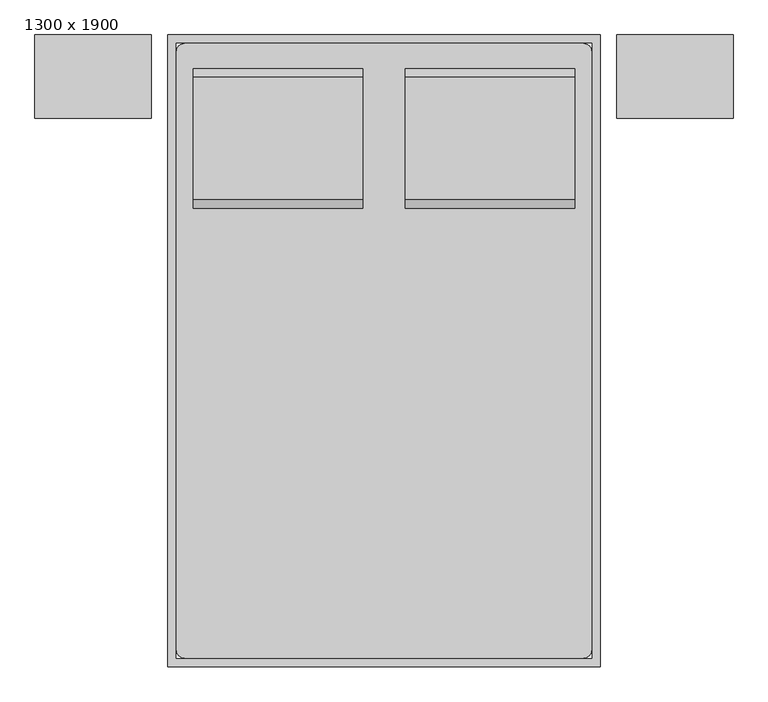
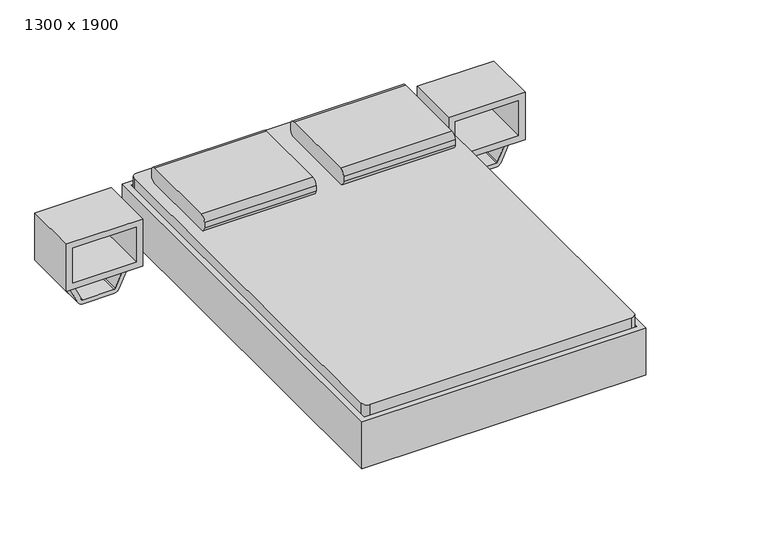
"""IFC4 building model written with IfcOpenShell, lengths in millimetres: furniture geometry, 双人床带床头柜 : 1300 x 1900."""

import ifcopenshell
import ifcopenshell.guid

model = None  # the IFC model being written
_history = None  # IfcOwnerHistory: only IFC2X3 demands one
_inside = {}  # id of a spatial element -> (the spatial element, [elements in it])
_under = {}  # id of a project, library or spatial element -> (it, [spatial elements below it])
_declared = {}  # id of a project -> (the project, [libraries it declares])
_typed = {}  # id of a type object -> (the type object, [elements of that type])
_made_of = {}  # id of a material, layer set ... -> (it, [elements and type objects made of it])


def new_model(schema):
    """Start an empty IFC model of exactly this schema.

    Asked for "IFC4X3", IfcOpenShell would pick the latest addendum, in which some entities
    have other attributes; the version numbers below select the first issue.
    IFC2X3 requires an IfcOwnerHistory on every rooted entity: one is made here for all.
    """
    global model, _history
    if schema == "IFC4X3":
        model = ifcopenshell.file(schema_version=(4, 3, 0, 0))
    else:
        model = ifcopenshell.file(schema=schema)
    _inside.clear()
    _under.clear()
    _declared.clear()
    _typed.clear()
    _made_of.clear()
    _history = None
    if model.schema == "IFC2X3":
        org = make("IfcOrganization", Name="unknown")
        user = make(
            "IfcPersonAndOrganization",
            ThePerson=make("IfcPerson", FamilyName="unknown"),
            TheOrganization=org,
        )
        app = make(
            "IfcApplication",
            ApplicationDeveloper=org,
            Version="unknown",
            ApplicationFullName="unknown",
            ApplicationIdentifier="unknown",
        )
        _history = make(
            "IfcOwnerHistory",
            OwningUser=user,
            OwningApplication=app,
            ChangeAction="ADDED",
            CreationDate=0,
        )
    return model


def make(cls, **values):
    """One entity of the class cls with the attributes given. An attribute that is None is left unset."""
    return model.create_entity(
        cls, **{name: value for name, value in values.items() if value is not None}
    )


def rooted(cls, **values):
    """An entity with a GlobalId (a new one), such as an element, a storey or a relation."""
    return make(cls, GlobalId=ifcopenshell.guid.new(), OwnerHistory=_history, **values)


def si_unit(unit_type, name, prefix=None):
    """IfcSIUnit, for example si_unit("LENGTHUNIT", "METRE", prefix="MILLI")."""
    return make("IfcSIUnit", UnitType=unit_type, Prefix=prefix, Name=name)


def assignment(units):
    """IfcUnitAssignment: the units of a project."""
    return None if units is None else make("IfcUnitAssignment", Units=units)


def point(xyz):
    """IfcCartesianPoint."""
    return None if xyz is None else make("IfcCartesianPoint", Coordinates=xyz)


def direction(xyz):
    """IfcDirection."""
    return None if xyz is None else make("IfcDirection", DirectionRatios=xyz)


def frame(location, z_axis=None, x_axis=None):
    """IfcAxis2Placement3D, a coordinate frame: its origin and axes. An axis left out is left unset."""
    return make(
        "IfcAxis2Placement3D",
        Location=point(location),
        Axis=direction(z_axis),
        RefDirection=direction(x_axis),
    )


def frame_2d(location, x_axis=None):
    """IfcAxis2Placement2D, a coordinate frame in the plane: its origin and x axis."""
    return make(
        "IfcAxis2Placement2D", Location=point(location), RefDirection=direction(x_axis)
    )


def origin():
    """The frame at (0, 0, 0) with its axes left unset."""
    return frame((0.0, 0.0, 0.0))


def place(relative_to, where):
    """IfcLocalPlacement: puts the frame where relative to a parent placement (None: the world)."""
    return make(
        "IfcLocalPlacement", PlacementRelTo=relative_to, RelativePlacement=where
    )


def context(
    kind, dimensions, precision=None, world=None, true_north=None, identifier=None
):
    """IfcGeometricRepresentationContext, for example the 3D "Model" context."""
    return make(
        "IfcGeometricRepresentationContext",
        ContextIdentifier=identifier,
        ContextType=kind,
        CoordinateSpaceDimension=dimensions,
        Precision=precision,
        WorldCoordinateSystem=world,
        TrueNorth=true_north,
    )


def project(units=None, contexts=None):
    """IfcProject with its units and contexts."""
    return rooted(
        "IfcProject",
        Name="project",
        RepresentationContexts=contexts,
        UnitsInContext=assignment(units),
    )


def spatial(cls, under=None, at=None, **own):
    """A site, building, storey or space (cls), placed at a placement, below another one or the project."""
    s = rooted(cls, ObjectPlacement=at, **own)
    if under is not None:
        _under.setdefault(under.id(), (under, []))[1].append(s)
    return s


def polyline(points):
    """IfcPolyline through the points."""
    return make("IfcPolyline", Points=[point(p) for p in points])


def circle_curve(where, radius):
    """IfcCircle in the frame where."""
    return make("IfcCircle", Position=where, Radius=radius)


def trimmed(basis, trim1, trim2, sense, master):
    """IfcTrimmedCurve: the piece of a basis curve between two trims."""
    return make(
        "IfcTrimmedCurve",
        BasisCurve=basis,
        Trim1=trim1,
        Trim2=trim2,
        SenseAgreement=sense,
        MasterRepresentation=master,
    )


def segment(curve, same_sense, transition):
    """IfcCompositeCurveSegment."""
    return make(
        "IfcCompositeCurveSegment",
        Transition=transition,
        SameSense=same_sense,
        ParentCurve=curve,
    )


def composite_curve(segments, self_intersect=None):
    """IfcCompositeCurve: segments joined end to end."""
    return make("IfcCompositeCurve", Segments=segments, SelfIntersect=self_intersect)


def outline(outer, holes=None, kind="AREA"):
    """IfcArbitraryClosedProfileDef: a profile drawn as a closed curve; with holes, ...WithVoids."""
    if holes is None:
        return make("IfcArbitraryClosedProfileDef", ProfileType=kind, OuterCurve=outer)
    return make(
        "IfcArbitraryProfileDefWithVoids",
        ProfileType=kind,
        OuterCurve=outer,
        InnerCurves=holes,
    )


def extrude(swept, where, along, depth):
    """IfcExtrudedAreaSolid: the profile swept, set in the frame where, extruded along a direction by depth."""
    return make(
        "IfcExtrudedAreaSolid",
        SweptArea=swept,
        Position=where,
        ExtrudedDirection=direction(along),
        Depth=depth,
    )


def shape(context_of_items, identifier, shape_type, items):
    """IfcShapeRepresentation: the items that make up one representation, for example the "Body"."""
    return make(
        "IfcShapeRepresentation",
        ContextOfItems=context_of_items,
        RepresentationIdentifier=identifier,
        RepresentationType=shape_type,
        Items=items,
    )


def source(mapping_origin, context_of_items, identifier, shape_type, items):
    """IfcRepresentationMap: a shape defined once, which mapped items show again and again."""
    return make(
        "IfcRepresentationMap",
        MappingOrigin=mapping_origin,
        MappedRepresentation=shape(context_of_items, identifier, shape_type, items),
    )


def transform(
    local_origin,
    x_axis=None,
    y_axis=None,
    z_axis=None,
    scale=None,
    scale2=None,
    scale3=None,
    uniform=True,
):
    """IfcCartesianTransformationOperator3D, or its non-uniform kind. x_axis, y_axis, z_axis: its Axis1, 2, 3."""
    if uniform:
        return make(
            "IfcCartesianTransformationOperator3D",
            Axis1=direction(x_axis),
            Axis2=direction(y_axis),
            LocalOrigin=point(local_origin),
            Scale=scale,
            Axis3=direction(z_axis),
        )
    return make(
        "IfcCartesianTransformationOperator3DnonUniform",
        Axis1=direction(x_axis),
        Axis2=direction(y_axis),
        LocalOrigin=point(local_origin),
        Scale=scale,
        Axis3=direction(z_axis),
        Scale2=scale2,
        Scale3=scale3,
    )


def mapped(mapping_source, mapping_target):
    """IfcMappedItem: shows the shape of a source again, moved by a transform."""
    return make(
        "IfcMappedItem", MappingSource=mapping_source, MappingTarget=mapping_target
    )


def made_of(thing, what):
    """Note that an element or type object is made of a material, layer set ...; save() writes the relation."""
    if what is not None:
        _made_of.setdefault(what.id(), (what, []))[1].append(thing)
    return thing


def element(
    cls,
    number,
    at=None,
    inside=None,
    cuts=None,
    type_object=None,
    material=None,
    context=None,
    identifier="Body",
    shape_type=None,
    held_by="IfcProductDefinitionShape",
    body=None,
    shapes=None,
    **own,
):
    """One element of the class cls, such as IfcWall. Its Tag is "e" and its number.

    at: its placement. inside: the storey or other place that contains it. cuts: it is an
    opening in that element (IfcRelVoidsElement). A single representation is given by context,
    identifier, shape_type and body (its items); several are given by shapes. held_by: the class
    of the entity that holds the representations. save() writes the other relations.
    """
    e = rooted(cls, Tag="e%d" % number, ObjectPlacement=at, **own)
    if body is not None:
        shapes = [shape(context, identifier, shape_type, body)]
    if shapes is not None:
        e.Representation = make(held_by, Representations=shapes)
    if inside is not None:
        _inside.setdefault(inside.id(), (inside, []))[1].append(e)
    if cuts is not None:
        rooted(
            "IfcRelVoidsElement", RelatingBuildingElement=cuts, RelatedOpeningElement=e
        )
    if type_object is not None:
        _typed.setdefault(type_object.id(), (type_object, []))[1].append(e)
    return made_of(e, material)


def aggregate(whole, parts):
    """IfcRelAggregates: a whole, such as a stair, and the parts it consists of."""
    return rooted("IfcRelAggregates", RelatingObject=whole, RelatedObjects=parts)


def save(model, path):
    """Write the relations noted so far, then the file.

    IfcRelAggregates (storeys below a building ...), IfcRelContainedInSpatialStructure (elements
    in a storey), IfcRelDefinesByType, IfcRelAssociatesMaterial and IfcRelDeclares: one each for
    every whole, place, type object, material and project.
    """
    for whole, parts in _under.values():
        aggregate(whole, parts)
    for where, things in _inside.values():
        rooted(
            "IfcRelContainedInSpatialStructure",
            RelatedElements=things,
            RelatingStructure=where,
        )
    for kind, things in _typed.values():
        rooted("IfcRelDefinesByType", RelatedObjects=things, RelatingType=kind)
    for what, things in _made_of.values():
        rooted("IfcRelAssociatesMaterial", RelatedObjects=things, RelatingMaterial=what)
    for by, libraries in _declared.values():
        rooted("IfcRelDeclares", RelatingContext=by, RelatedDefinitions=libraries)
    model.write(path)


def plane_surface(at):
    """IfcPlane: the flat surface through the origin of the frame at, square to its z axis."""
    return make("IfcPlane", Position=at)


def cylinder_surface(at, radius):
    """IfcCylindricalSurface: all points at the distance radius from the z axis of the frame at."""
    return make("IfcCylindricalSurface", Position=at, Radius=radius)


def revolved_surface(curve, axis_point, axis_direction):
    """IfcSurfaceOfRevolution: the curve turned about the line through axis_point along axis_direction."""
    return make(
        "IfcSurfaceOfRevolution",
        SweptCurve=make("IfcArbitraryOpenProfileDef", ProfileType="CURVE", Curve=curve),
        AxisPosition=make("IfcAxis1Placement", Location=point(axis_point), Axis=direction(axis_direction)),
    )


def advanced_brep(points, edges, surfaces, faces):
    """IfcAdvancedBrep: a solid bounded by faces that lie on surfaces and meet in shared edges.

    An edge is (start, end): straight between two places in points (the first is 0);
    or (start, end, curve); or (start, end, curve, False) where it runs against its curve.
    A face is (place in surfaces, loops), or (place, loops, False) where it looks against
    its surface's normal. A loop lists edges by number (the first is 1), with a minus sign
    where the edge is run from its end to its start. The first loop is the outer one.
    """
    corners = [point(p) for p in points]
    vertices = [make("IfcVertexPoint", VertexGeometry=c) for c in corners]
    made = []
    for start, end, *more in edges:
        made.append(
            make(
                "IfcEdgeCurve",
                EdgeStart=vertices[start],
                EdgeEnd=vertices[end],
                EdgeGeometry=more[0] if more else make("IfcPolyline", Points=[corners[start], corners[end]]),
                SameSense=more[1] if len(more) > 1 else True,
            )
        )
    hull = []
    for where, loops, *sense in faces:
        bounds = []
        for j, loop in enumerate(loops):
            ring = [make("IfcOrientedEdge", EdgeElement=made[abs(k) - 1], Orientation=k > 0) for k in loop]
            bounds.append(
                make(
                    "IfcFaceOuterBound" if j == 0 else "IfcFaceBound",
                    Bound=make("IfcEdgeLoop", EdgeList=ring),
                    Orientation=True,
                )
            )
        hull.append(make("IfcAdvancedFace", Bounds=bounds, FaceSurface=surfaces[where], SameSense=sense[0] if sense else True))
    return make("IfcAdvancedBrep", Outer=make("IfcClosedShell", CfsFaces=hull))


def furniture_1300_x_1900_48583a1e(model_context):
    return source(origin(), model_context, "Body", "SolidModel", [
        advanced_brep(
        [(-285.1231784, 461.5704918, 177.8), (-285.1231784, 385.3704918, 177.8), (-285.1231784, 385.3704918, 196.85), (-285.1231784, 461.5704918, 196.85), (-234.3231784, 461.5704918, 177.8), (-234.3231784, 385.3704918, 177.8), (-222.1869899, 385.3704918, 196.85), (-222.1869899, 461.5704918, 196.85), (-158.2523099, 461.5704918, 14.6654962), (-158.2523099, 385.3704918, 14.6654962), (-140.9871466, 385.3704918, 22.716374), (-140.9871466, 461.5704918, 22.716374), (-135.2320921, 385.3704918, 0.0), (-135.2320921, 461.5704918, 0.0), (-135.2320921, 385.3704918, 19.05), (-135.2320921, 461.5704918, 19.05), (-56.6195862, 461.5704918, 0.0), (-56.6195862, 385.3704918, 0.0), (-56.6195862, 385.3704918, 19.05), (-56.6195862, 461.5704918, 19.05), (-43.9195862, 385.3704918, 3.4029547), (-43.9195862, 461.5704918, 3.4029547), (-53.4445862, 385.3704918, 19.9007387), (-53.4445862, 461.5704918, 19.9007387), (16.177459, 461.5704918, 38.1), (16.177459, 385.3704918, 38.1), (11.0730269, 385.3704918, 57.15), (11.0730269, 461.5704918, 57.15), (662.4518216, 461.5704918, 38.1), (662.4518216, 385.3704918, 38.1), (667.5562537, 385.3704918, 57.15), (667.5562537, 461.5704918, 57.15), (722.5488669, 461.5704918, 3.4029547), (722.5488669, 385.3704918, 3.4029547), (732.0738669, 385.3704918, 19.9007387), (732.0738669, 461.5704918, 19.9007387), (735.2488669, 385.3704918, 0.0), (735.2488669, 461.5704918, 0.0), (735.2488669, 385.3704918, 19.05), (735.2488669, 461.5704918, 19.05), (813.8613728, 461.5704918, 0.0), (813.8613728, 385.3704918, 0.0), (813.8613728, 385.3704918, 19.05), (813.8613728, 461.5704918, 19.05), (836.8815906, 385.3704918, 14.6654962), (836.8815906, 461.5704918, 14.6654962), (819.6164272, 385.3704918, 22.716374), (819.6164272, 461.5704918, 22.716374), (912.952459, 461.5704918, 177.8), (912.952459, 385.3704918, 177.8), (900.8162705, 385.3704918, 196.85), (900.8162705, 461.5704918, 196.85), (963.752459, 461.5704918, 177.8), (963.752459, 461.5704918, 196.85), (963.752459, 385.3704918, 196.85), (963.752459, 385.3704918, 177.8)],
        [
            (0, 1),
            (1, 2),
            (2, 3),
            (3, 0),
            (0, 4),
            (4, 5),
            (5, 1),
            (5, 6),
            (6, 2),
            (6, 7),
            (7, 3),
            (7, 4),
            (4, 8),
            (8, 9),
            (9, 5),
            (9, 10),
            (10, 6),
            (10, 11),
            (11, 7),
            (11, 8),
            (12, 9, circle_curve(frame((-135.2320921, 385.3704918, 25.4), z_axis=(0.0, 1.0, 0.0), x_axis=(-0.9063077870366494, 0.0, -0.4226182617407007)), 25.4)),
            (8, 13, circle_curve(frame((-135.2320921, 461.5704918, 25.4), z_axis=(0.0, -1.0, 0.0), x_axis=(-0.9063077870366494, 0.0, -0.4226182617407007)), 25.4)),
            (13, 12),
            (14, 10, circle_curve(frame((-135.2320921, 385.3704918, 25.4), z_axis=(0.0, 1.0, 0.0), x_axis=(-0.9063077870366494, 0.0, -0.4226182617407007)), 6.35)),
            (12, 14),
            (15, 11, circle_curve(frame((-135.2320921, 461.5704918, 25.4), z_axis=(0.0, 1.0, 0.0), x_axis=(-0.9063077870366494, 0.0, -0.4226182617407007)), 6.35)),
            (14, 15),
            (15, 13),
            (13, 16),
            (16, 17),
            (17, 12),
            (17, 18),
            (18, 14),
            (18, 19),
            (19, 15),
            (19, 16),
            (20, 17, circle_curve(frame((-56.6195862, 385.3704918, 25.4), z_axis=(0.0, 1.0, 0.0), x_axis=(0.0, 0.0, -1.0)), 25.4)),
            (16, 21, circle_curve(frame((-56.6195862, 461.5704918, 25.4), z_axis=(0.0, -1.0, 0.0), x_axis=(0.0, 0.0, -1.0)), 25.4)),
            (21, 20),
            (22, 18, circle_curve(frame((-56.6195862, 385.3704918, 25.4), z_axis=(0.0, 1.0, 0.0), x_axis=(0.0, 0.0, -1.0)), 6.35)),
            (20, 22),
            (23, 19, circle_curve(frame((-56.6195862, 461.5704918, 25.4), z_axis=(0.0, 1.0, 0.0), x_axis=(0.0, 0.0, -1.0)), 6.35)),
            (22, 23),
            (23, 21),
            (21, 24),
            (24, 25),
            (25, 20),
            (25, 26),
            (26, 22),
            (26, 27),
            (27, 23),
            (27, 24),
            (24, 28),
            (28, 29),
            (29, 25),
            (29, 30),
            (30, 26),
            (30, 31),
            (31, 27),
            (31, 28),
            (28, 32),
            (32, 33),
            (33, 29),
            (33, 34),
            (34, 30),
            (34, 35),
            (35, 31),
            (35, 32),
            (36, 33, circle_curve(frame((735.2488669, 385.3704918, 25.4), z_axis=(0.0, 1.0, 0.0), x_axis=(-0.5000000000000505, 0.0, -0.8660254037844094)), 25.4)),
            (32, 37, circle_curve(frame((735.2488669, 461.5704918, 25.4), z_axis=(0.0, -1.0, 0.0), x_axis=(-0.5000000000000505, 0.0, -0.8660254037844094)), 25.4)),
            (37, 36),
            (38, 34, circle_curve(frame((735.2488669, 385.3704918, 25.4), z_axis=(0.0, 1.0, 0.0), x_axis=(-0.5000000000000505, 0.0, -0.8660254037844094)), 6.35)),
            (36, 38),
            (39, 35, circle_curve(frame((735.2488669, 461.5704918, 25.4), z_axis=(0.0, 1.0, 0.0), x_axis=(-0.5000000000000505, 0.0, -0.8660254037844094)), 6.35)),
            (38, 39),
            (39, 37),
            (37, 40),
            (40, 41),
            (41, 36),
            (41, 42),
            (42, 38),
            (42, 43),
            (43, 39),
            (43, 40),
            (44, 41, circle_curve(frame((813.8613728, 385.3704918, 25.4), z_axis=(0.0, 1.0, 0.0), x_axis=(0.0, 0.0, -1.0)), 25.4)),
            (40, 45, circle_curve(frame((813.8613728, 461.5704918, 25.4), z_axis=(0.0, -1.0, 0.0), x_axis=(0.0, 0.0, -1.0)), 25.4)),
            (45, 44),
            (46, 42, circle_curve(frame((813.8613728, 385.3704918, 25.4), z_axis=(0.0, 1.0, 0.0), x_axis=(0.0, 0.0, -1.0)), 6.35)),
            (44, 46),
            (47, 43, circle_curve(frame((813.8613728, 461.5704918, 25.4), z_axis=(0.0, 1.0, 0.0), x_axis=(0.0, 0.0, -1.0)), 6.35)),
            (46, 47),
            (47, 45),
            (45, 48),
            (48, 49),
            (49, 44),
            (49, 50),
            (50, 46),
            (50, 51),
            (51, 47),
            (51, 48),
            (52, 53),
            (53, 54),
            (54, 55),
            (55, 52),
            (48, 52),
            (55, 49),
            (54, 50),
            (53, 51),
        ],
        [
            plane_surface(frame((-285.1231784, 715.5704918, -152.9490627), z_axis=(-1.0, 0.0, 0.0), x_axis=(0.0, 1.0, 0.0))),
            plane_surface(frame((-285.1231784, 461.5704918, 177.8), z_axis=(0.0, 0.0, -1.0), x_axis=(1.0, 0.0, 0.0))),
            plane_surface(frame((-285.1231784, 385.3704918, 177.8), z_axis=(0.0, -1.0, 0.0), x_axis=(1.0, 0.0, 0.0))),
            plane_surface(frame((-285.1231784, 385.3704918, 196.85), z_axis=(0.0, 0.0, 1.0), x_axis=(1.0, 0.0, 0.0))),
            plane_surface(frame((-285.1231784, 461.5704918, 196.85), z_axis=(0.0, 1.0, 0.0), x_axis=(1.0, 0.0, 0.0))),
            plane_surface(frame((-234.3231784, 461.5704918, 177.8), z_axis=(-0.9063077870366483, 0.0, -0.42261826174070305), x_axis=(0.42261826174070305, 0.0, -0.9063077870366483))),
            plane_surface(frame((-234.3231784, 385.3704918, 177.8), z_axis=(0.0, -1.0, 0.0), x_axis=(0.4226182617407031, 0.0, -0.9063077870366483))),
            plane_surface(frame((-222.1869899, 385.3704918, 196.85), z_axis=(0.9063077870366483, 0.0, 0.42261826174070316), x_axis=(0.42261826174070316, 0.0, -0.9063077870366483))),
            plane_surface(frame((-222.1869899, 461.5704918, 196.85), z_axis=(0.0, 1.0, 0.0), x_axis=(0.42261826174070316, 0.0, -0.9063077870366483))),
            cylinder_surface(frame((-135.2320921, 715.5704918, 25.4), z_axis=(0.0, -1.0, 0.0), x_axis=(-0.9063077870366494, 0.0, -0.4226182617407007)), 25.4),
            plane_surface(frame((-135.2320921, 385.3704918, 25.4), z_axis=(0.0, -1.0, 0.0), x_axis=(-0.9063077870366494, 0.0, -0.4226182617407007))),
            revolved_surface(polyline([(-140.9871465476827, 385.3704918, 22.71637403794655), (-140.9871465476827, 461.5704918, 22.71637403794655)]), (-135.2320921, 715.5704918, 25.4), (0.0, -1.0, 0.0)),
            plane_surface(frame((-135.2320921, 461.5704918, 25.4), z_axis=(0.0, 1.0, 0.0), x_axis=(-0.9063077870366494, 0.0, -0.4226182617407007))),
            plane_surface(frame((-135.2320921, 461.5704918, 0.0), z_axis=(0.0, 0.0, -1.0), x_axis=(1.0, 0.0, 0.0))),
            plane_surface(frame((-135.2320921, 385.3704918, 0.0), z_axis=(0.0, -1.0, 0.0), x_axis=(1.0, 0.0, 0.0))),
            plane_surface(frame((-135.2320921, 385.3704918, 19.05), z_axis=(0.0, 0.0, 1.0), x_axis=(1.0, 0.0, 0.0))),
            plane_surface(frame((-135.2320921, 461.5704918, 19.05), z_axis=(0.0, 1.0, 0.0), x_axis=(1.0, 0.0, 0.0))),
            cylinder_surface(frame((-56.6195862, 715.5704918, 25.4), z_axis=(0.0, -1.0, 0.0), x_axis=(0.0, 0.0, -1.0)), 25.4),
            plane_surface(frame((-56.6195862, 385.3704918, 25.4), z_axis=(0.0, -1.0, 0.0), x_axis=(0.0, 0.0, -1.0))),
            revolved_surface(polyline([(-56.6195862, 385.3704918, 19.049999999999997), (-56.6195862, 461.5704918, 19.049999999999997)]), (-56.6195862, 715.5704918, 25.4), (0.0, -1.0, 0.0)),
            plane_surface(frame((-56.6195862, 461.5704918, 25.4), z_axis=(0.0, 1.0, 0.0), x_axis=(0.0, 0.0, -1.0))),
            plane_surface(frame((-43.9195862, 461.5704918, 3.4029547), z_axis=(0.49999999999987826, 0.0, -0.8660254037845089), x_axis=(0.8660254037845089, 0.0, 0.49999999999987826))),
            plane_surface(frame((-43.9195862, 385.3704918, 3.4029547), z_axis=(0.0, -1.0, 0.0), x_axis=(0.866025403784509, 0.0, 0.49999999999987815))),
            plane_surface(frame((-53.4445862, 385.3704918, 19.9007387), z_axis=(-0.49999999999987926, 0.0, 0.8660254037845083), x_axis=(0.8660254037845083, 0.0, 0.49999999999987926))),
            plane_surface(frame((-53.4445862, 461.5704918, 19.9007387), z_axis=(0.0, 1.0, 0.0), x_axis=(0.8660254037845087, 0.0, 0.4999999999998789))),
            plane_surface(frame((16.177459, 461.5704918, 38.1), z_axis=(0.0, 0.0, -1.0), x_axis=(1.0, 0.0, 0.0))),
            plane_surface(frame((16.177459, 385.3704918, 38.1), z_axis=(0.0, -1.0, 0.0), x_axis=(1.0, 0.0, 0.0))),
            plane_surface(frame((11.0730269, 385.3704918, 57.15), z_axis=(0.0, 0.0, 1.0), x_axis=(1.0, 0.0, 0.0))),
            plane_surface(frame((11.0730269, 461.5704918, 57.15), z_axis=(0.0, 1.0, 0.0), x_axis=(1.0, 0.0, 0.0))),
            plane_surface(frame((662.4518216, 461.5704918, 38.1), z_axis=(-0.5000000000000518, 0.0, -0.8660254037844087), x_axis=(0.8660254037844087, 0.0, -0.5000000000000518))),
            plane_surface(frame((662.4518216, 385.3704918, 38.1), z_axis=(0.0, -1.0, 0.0), x_axis=(0.8660254037844093, 0.0, -0.500000000000051))),
            plane_surface(frame((667.5562537, 385.3704918, 57.15), z_axis=(0.5000000000000507, 0.0, 0.8660254037844094), x_axis=(0.8660254037844094, 0.0, -0.5000000000000507))),
            plane_surface(frame((667.5562537, 461.5704918, 57.15), z_axis=(0.0, 1.0000000000000002, 0.0), x_axis=(0.8660254037844094, 0.0, -0.5000000000000508))),
            cylinder_surface(frame((735.2488669, 715.5704918, 25.4), z_axis=(0.0, -1.0, 0.0), x_axis=(-0.5000000000000505, 0.0, -0.8660254037844094)), 25.4),
            plane_surface(frame((735.2488669, 385.3704918, 25.4), z_axis=(0.0, -1.0, 0.0), x_axis=(-0.5000000000000506, 0.0, -0.8660254037844095))),
            revolved_surface(polyline([(732.0738668999998, 385.3704918, 19.900738685969), (732.0738668999998, 461.5704918, 19.900738685969)]), (735.2488669, 715.5704918, 25.4), (0.0, -1.0, 0.0)),
            plane_surface(frame((735.2488669, 461.5704918, 25.4), z_axis=(0.0, 1.0, 0.0), x_axis=(-0.5000000000000506, 0.0, -0.8660254037844095))),
            plane_surface(frame((735.2488669, 461.5704918, 0.0), z_axis=(0.0, 0.0, -1.0), x_axis=(1.0, 0.0, 0.0))),
            plane_surface(frame((735.2488669, 385.3704918, 0.0), z_axis=(0.0, -1.0, 0.0), x_axis=(1.0, 0.0, 0.0))),
            plane_surface(frame((735.2488669, 385.3704918, 19.05), z_axis=(0.0, 0.0, 1.0), x_axis=(1.0, 0.0, 0.0))),
            plane_surface(frame((735.2488669, 461.5704918, 19.05), z_axis=(0.0, 1.0, 0.0), x_axis=(1.0, 0.0, 0.0))),
            cylinder_surface(frame((813.8613728, 715.5704918, 25.4), z_axis=(0.0, -1.0, 0.0), x_axis=(0.0, 0.0, -1.0)), 25.4),
            plane_surface(frame((813.8613728, 385.3704918, 25.4), z_axis=(0.0, -1.0, 0.0), x_axis=(0.0, 0.0, -1.0))),
            revolved_surface(polyline([(813.8613728, 385.3704918, 19.049999999999997), (813.8613728, 461.5704918, 19.049999999999997)]), (813.8613728, 715.5704918, 25.4), (0.0, -1.0, 0.0)),
            plane_surface(frame((813.8613728, 461.5704918, 25.4), z_axis=(0.0, 1.0, 0.0), x_axis=(0.0, 0.0, -1.0))),
            plane_surface(frame((836.8815906, 461.5704918, 14.6654962), z_axis=(0.9063077870366775, 0.0, -0.42261826174064077), x_axis=(0.42261826174064077, 0.0, 0.9063077870366775))),
            plane_surface(frame((836.8815906, 385.3704918, 14.6654962), z_axis=(0.0, -1.0, 0.0), x_axis=(0.42261826174063993, 0.0, 0.9063077870366777))),
            plane_surface(frame((819.6164272, 385.3704918, 22.716374), z_axis=(-0.9063077870366776, 0.0, 0.4226182617406402), x_axis=(0.4226182617406402, 0.0, 0.9063077870366776))),
            plane_surface(frame((819.6164272, 461.5704918, 22.716374), z_axis=(0.0, 1.0, 0.0), x_axis=(0.4226182617406405, 0.0, 0.9063077870366775))),
            plane_surface(frame((963.752459, 715.5704918, -152.9490627), z_axis=(1.0, 0.0, 0.0), x_axis=(0.0, 1.0, 0.0))),
            plane_surface(frame((912.952459, 461.5704918, 177.8), z_axis=(0.0, 0.0, -1.0), x_axis=(1.0, 0.0, 0.0))),
            plane_surface(frame((912.952459, 385.3704918, 177.8), z_axis=(0.0, -1.0, 0.0), x_axis=(1.0, 0.0, 0.0))),
            plane_surface(frame((900.8162705, 385.3704918, 196.85), z_axis=(0.0, 0.0, 1.0), x_axis=(1.0, 0.0, 0.0))),
            plane_surface(frame((900.8162705, 461.5704918, 196.85), z_axis=(0.0, 1.0, 0.0), x_axis=(1.0, 0.0, 0.0))),
        ],
        [
            (0, [[1, 2, 3, 4]]),
            (1, [[-1, 5, 6, 7]]),
            (2, [[-2, -7, 8, 9]]),
            (3, [[-3, -9, 10, 11]]),
            (4, [[-4, -11, 12, -5]]),
            (5, [[-6, 13, 14, 15]]),
            (6, [[-8, -15, 16, 17]]),
            (7, [[-10, -17, 18, 19]]),
            (8, [[-12, -19, 20, -13]]),
            (9, [[21, -14, 22, 23]]),
            (10, [[24, -16, -21, 25]]),
            (11, [[26, -18, -24, 27]]),
            (12, [[-22, -20, -26, 28]]),
            (13, [[-23, 29, 30, 31]]),
            (14, [[-25, -31, 32, 33]]),
            (15, [[-27, -33, 34, 35]]),
            (16, [[-28, -35, 36, -29]]),
            (17, [[37, -30, 38, 39]]),
            (18, [[40, -32, -37, 41]]),
            (19, [[42, -34, -40, 43]]),
            (20, [[-38, -36, -42, 44]]),
            (21, [[-39, 45, 46, 47]]),
            (22, [[-41, -47, 48, 49]]),
            (23, [[-43, -49, 50, 51]]),
            (24, [[-44, -51, 52, -45]]),
            (25, [[-46, 53, 54, 55]]),
            (26, [[-48, -55, 56, 57]]),
            (27, [[-50, -57, 58, 59]]),
            (28, [[-52, -59, 60, -53]]),
            (29, [[-54, 61, 62, 63]]),
            (30, [[-56, -63, 64, 65]]),
            (31, [[-58, -65, 66, 67]]),
            (32, [[-60, -67, 68, -61]]),
            (33, [[69, -62, 70, 71]]),
            (34, [[72, -64, -69, 73]]),
            (35, [[74, -66, -72, 75]]),
            (36, [[-70, -68, -74, 76]]),
            (37, [[-71, 77, 78, 79]]),
            (38, [[-73, -79, 80, 81]]),
            (39, [[-75, -81, 82, 83]]),
            (40, [[-76, -83, 84, -77]]),
            (41, [[85, -78, 86, 87]]),
            (42, [[88, -80, -85, 89]]),
            (43, [[90, -82, -88, 91]]),
            (44, [[-86, -84, -90, 92]]),
            (45, [[-87, 93, 94, 95]]),
            (46, [[-89, -95, 96, 97]]),
            (47, [[-91, -97, 98, 99]]),
            (48, [[-92, -99, 100, -93]]),
            (49, [[101, 102, 103, 104]]),
            (50, [[-94, 105, -104, 106]]),
            (51, [[-96, -106, -103, 107]]),
            (52, [[-98, -107, -102, 108]]),
            (53, [[-100, -108, -101, -105]]),
        ],
    ),
        advanced_brep(
        [(-285.447541, -879.6295082, 196.85), (-285.447541, -879.6295082, 177.8), (-285.447541, -955.8295082, 177.8), (-285.447541, -955.8295082, 196.85), (-222.5113525, -879.6295082, 196.85), (-234.647541, -879.6295082, 177.8), (-234.647541, -955.8295082, 177.8), (-222.5113525, -955.8295082, 196.85), (-141.3115092, -879.6295082, 22.716374), (-158.5766725, -879.6295082, 14.6654962), (-158.5766725, -955.8295082, 14.6654962), (-141.3115092, -955.8295082, 22.716374), (-135.5564547, -879.6295082, 0.0), (-135.5564547, -879.6295082, 19.05), (-135.5564547, -955.8295082, 0.0), (-135.5564547, -955.8295082, 19.05), (-56.9439489, -879.6295082, 19.05), (-56.9439489, -879.6295082, 0.0), (-56.9439489, -955.8295082, 0.0), (-56.9439489, -955.8295082, 19.05), (-44.2439489, -879.6295082, 3.4029547), (-53.7689489, -879.6295082, 19.9007387), (-44.2439489, -955.8295082, 3.4029547), (-53.7689489, -955.8295082, 19.9007387), (10.7486643, -879.6295082, 57.15), (15.8530964, -879.6295082, 38.1), (15.8530964, -955.8295082, 38.1), (10.7486643, -955.8295082, 57.15), (667.5562537, -879.6295082, 57.15), (662.4518216, -879.6295082, 38.1), (662.4518216, -955.8295082, 38.1), (667.5562537, -955.8295082, 57.15), (732.0738669, -879.6295082, 19.9007387), (722.5488669, -879.6295082, 3.4029547), (722.5488669, -955.8295082, 3.4029547), (732.0738669, -955.8295082, 19.9007387), (735.2488669, -879.6295082, 0.0), (735.2488669, -879.6295082, 19.05), (735.2488669, -955.8295082, 0.0), (735.2488669, -955.8295082, 19.05), (813.8613728, -879.6295082, 19.05), (813.8613728, -879.6295082, 0.0), (813.8613728, -955.8295082, 0.0), (813.8613728, -955.8295082, 19.05), (836.8815906, -879.6295082, 14.6654962), (819.6164272, -879.6295082, 22.716374), (836.8815906, -955.8295082, 14.6654962), (819.6164272, -955.8295082, 22.716374), (900.8162705, -879.6295082, 196.85), (912.952459, -879.6295082, 177.8), (912.952459, -955.8295082, 177.8), (900.8162705, -955.8295082, 196.85), (963.752459, -879.6295082, 196.85), (963.752459, -955.8295082, 196.85), (963.752459, -955.8295082, 177.8), (963.752459, -879.6295082, 177.8)],
        [
            (0, 1),
            (1, 2),
            (2, 3),
            (3, 0),
            (0, 4),
            (4, 5),
            (5, 1),
            (5, 6),
            (6, 2),
            (6, 7),
            (7, 3),
            (7, 4),
            (4, 8),
            (8, 9),
            (9, 5),
            (9, 10),
            (10, 6),
            (10, 11),
            (11, 7),
            (11, 8),
            (12, 9, circle_curve(frame((-135.5564547, -879.6295082, 25.4), z_axis=(0.0, 1.0, 0.0), x_axis=(-0.9063077870366627, 0.0, -0.42261826174067213)), 25.4)),
            (8, 13, circle_curve(frame((-135.5564547, -879.6295082, 25.4), z_axis=(0.0, -1.0, 0.0), x_axis=(-0.9063077870366627, 0.0, -0.42261826174067213)), 6.35)),
            (13, 12),
            (14, 10, circle_curve(frame((-135.5564547, -955.8295082, 25.4), z_axis=(0.0, 1.0, 0.0), x_axis=(-0.9063077870366627, 0.0, -0.42261826174067213)), 25.4)),
            (12, 14),
            (15, 11, circle_curve(frame((-135.5564547, -955.8295082, 25.4), z_axis=(0.0, 1.0, 0.0), x_axis=(-0.9063077870366627, 0.0, -0.42261826174067213)), 6.35)),
            (14, 15),
            (15, 13),
            (13, 16),
            (16, 17),
            (17, 12),
            (17, 18),
            (18, 14),
            (18, 19),
            (19, 15),
            (19, 16),
            (20, 17, circle_curve(frame((-56.9439489, -879.6295082, 25.4), z_axis=(0.0, 1.0, 0.0), x_axis=(0.0, 0.0, -1.0)), 25.4)),
            (16, 21, circle_curve(frame((-56.9439489, -879.6295082, 25.4), z_axis=(0.0, -1.0, 0.0), x_axis=(0.0, 0.0, -1.0)), 6.35)),
            (21, 20),
            (22, 18, circle_curve(frame((-56.9439489, -955.8295082, 25.4), z_axis=(0.0, 1.0, 0.0), x_axis=(0.0, 0.0, -1.0)), 25.4)),
            (20, 22),
            (23, 19, circle_curve(frame((-56.9439489, -955.8295082, 25.4), z_axis=(0.0, 1.0, 0.0), x_axis=(0.0, 0.0, -1.0)), 6.35)),
            (22, 23),
            (23, 21),
            (21, 24),
            (24, 25),
            (25, 20),
            (25, 26),
            (26, 22),
            (26, 27),
            (27, 23),
            (27, 24),
            (24, 28),
            (28, 29),
            (29, 25),
            (29, 30),
            (30, 26),
            (30, 31),
            (31, 27),
            (31, 28),
            (28, 32),
            (32, 33),
            (33, 29),
            (33, 34),
            (34, 30),
            (34, 35),
            (35, 31),
            (35, 32),
            (36, 33, circle_curve(frame((735.2488669, -879.6295082, 25.4), z_axis=(0.0, 1.0, 0.0), x_axis=(-0.5000000000000517, 0.0, -0.8660254037844087)), 25.4)),
            (32, 37, circle_curve(frame((735.2488669, -879.6295082, 25.4), z_axis=(0.0, -1.0, 0.0), x_axis=(-0.5000000000000517, 0.0, -0.8660254037844087)), 6.35)),
            (37, 36),
            (38, 34, circle_curve(frame((735.2488669, -955.8295082, 25.4), z_axis=(0.0, 1.0, 0.0), x_axis=(-0.5000000000000517, 0.0, -0.8660254037844087)), 25.4)),
            (36, 38),
            (39, 35, circle_curve(frame((735.2488669, -955.8295082, 25.4), z_axis=(0.0, 1.0, 0.0), x_axis=(-0.5000000000000517, 0.0, -0.8660254037844087)), 6.35)),
            (38, 39),
            (39, 37),
            (37, 40),
            (40, 41),
            (41, 36),
            (41, 42),
            (42, 38),
            (42, 43),
            (43, 39),
            (43, 40),
            (44, 41, circle_curve(frame((813.8613728, -879.6295082, 25.4), z_axis=(0.0, 1.0, 0.0), x_axis=(0.0, 0.0, -1.0)), 25.4)),
            (40, 45, circle_curve(frame((813.8613728, -879.6295082, 25.4), z_axis=(0.0, -1.0, 0.0), x_axis=(0.0, 0.0, -1.0)), 6.35)),
            (45, 44),
            (46, 42, circle_curve(frame((813.8613728, -955.8295082, 25.4), z_axis=(0.0, 1.0, 0.0), x_axis=(0.0, 0.0, -1.0)), 25.4)),
            (44, 46),
            (47, 43, circle_curve(frame((813.8613728, -955.8295082, 25.4), z_axis=(0.0, 1.0, 0.0), x_axis=(0.0, 0.0, -1.0)), 6.35)),
            (46, 47),
            (47, 45),
            (45, 48),
            (48, 49),
            (49, 44),
            (49, 50),
            (50, 46),
            (50, 51),
            (51, 47),
            (51, 48),
            (52, 53),
            (53, 54),
            (54, 55),
            (55, 52),
            (48, 52),
            (55, 49),
            (54, 50),
            (53, 51),
        ],
        [
            plane_surface(frame((-285.447541, -1184.4295082, -127.5947323), z_axis=(-1.0, 0.0, 0.0), x_axis=(0.0, 1.0, 0.0))),
            plane_surface(frame((-285.447541, -879.6295082, 196.85), z_axis=(0.0, 1.0, 0.0), x_axis=(1.0, 0.0, 0.0))),
            plane_surface(frame((-285.447541, -879.6295082, 177.8), z_axis=(0.0, 0.0, -1.0), x_axis=(1.0, 0.0, 0.0))),
            plane_surface(frame((-285.447541, -955.8295082, 177.8), z_axis=(0.0, -1.0, 0.0), x_axis=(1.0, 0.0, 0.0))),
            plane_surface(frame((-285.447541, -955.8295082, 196.85), z_axis=(0.0, 0.0, 1.0), x_axis=(1.0, 0.0, 0.0))),
            plane_surface(frame((-222.5113525, -879.6295082, 196.85), z_axis=(0.0, 1.0, 0.0), x_axis=(0.42261826174067113, 0.0, -0.9063077870366631))),
            plane_surface(frame((-234.647541, -879.6295082, 177.8), z_axis=(-0.9063077870366633, 0.0, -0.422618261740671), x_axis=(0.422618261740671, 0.0, -0.9063077870366633))),
            plane_surface(frame((-234.647541, -955.8295082, 177.8), z_axis=(0.0, -1.0, 0.0), x_axis=(0.422618261740671, 0.0, -0.9063077870366633))),
            plane_surface(frame((-222.5113525, -955.8295082, 196.85), z_axis=(0.9063077870366631, 0.0, 0.42261826174067113), x_axis=(0.42261826174067113, 0.0, -0.9063077870366631))),
            plane_surface(frame((-135.5564547, -879.6295082, 25.4), z_axis=(0.0, 1.0, 0.0), x_axis=(-0.9063077870366627, 0.0, -0.42261826174067213))),
            cylinder_surface(frame((-135.5564547, -1184.4295082, 25.4), z_axis=(0.0, -1.0, 0.0), x_axis=(-0.9063077870366627, 0.0, -0.42261826174067213)), 25.4),
            plane_surface(frame((-135.5564547, -955.8295082, 25.4), z_axis=(0.0, -1.0, 0.0), x_axis=(-0.9063077870366627, 0.0, -0.42261826174067213))),
            revolved_surface(polyline([(-141.31150914768278, -955.8295082, 22.716374037946732), (-141.31150914768278, -879.6295082, 22.716374037946732)]), (-135.5564547, -1184.4295082, 25.4), (0.0, -1.0, 0.0)),
            plane_surface(frame((-135.5564547, -879.6295082, 19.05), z_axis=(0.0, 1.0, 0.0), x_axis=(1.0, 0.0, 0.0))),
            plane_surface(frame((-135.5564547, -879.6295082, 0.0), z_axis=(0.0, 0.0, -1.0), x_axis=(1.0, 0.0, 0.0))),
            plane_surface(frame((-135.5564547, -955.8295082, 0.0), z_axis=(0.0, -1.0, 0.0), x_axis=(1.0, 0.0, 0.0))),
            plane_surface(frame((-135.5564547, -955.8295082, 19.05), z_axis=(0.0, 0.0, 1.0), x_axis=(1.0, 0.0, 0.0))),
            plane_surface(frame((-56.9439489, -879.6295082, 25.4), z_axis=(0.0, 1.0, 0.0), x_axis=(0.0, 0.0, -1.0))),
            cylinder_surface(frame((-56.9439489, -1184.4295082, 25.4), z_axis=(0.0, -1.0, 0.0), x_axis=(0.0, 0.0, -1.0)), 25.4),
            plane_surface(frame((-56.9439489, -955.8295082, 25.4), z_axis=(0.0, -1.0, 0.0), x_axis=(0.0, 0.0, -1.0))),
            revolved_surface(polyline([(-56.9439489, -955.8295082, 19.049999999999997), (-56.9439489, -879.6295082, 19.049999999999997)]), (-56.9439489, -1184.4295082, 25.4), (0.0, -1.0, 0.0)),
            plane_surface(frame((-53.7689489, -879.6295082, 19.9007387), z_axis=(0.0, 1.0, 0.0), x_axis=(0.8660254037844793, 0.0, 0.4999999999999296))),
            plane_surface(frame((-44.2439489, -879.6295082, 3.4029547), z_axis=(0.4999999999999292, 0.0, -0.8660254037844796), x_axis=(0.8660254037844796, 0.0, 0.4999999999999292))),
            plane_surface(frame((-44.2439489, -955.8295082, 3.4029547), z_axis=(0.0, -1.0000000000000002, 0.0), x_axis=(0.8660254037844802, 0.0, 0.4999999999999281))),
            plane_surface(frame((-53.7689489, -955.8295082, 19.9007387), z_axis=(-0.49999999999992867, 0.0, 0.8660254037844798), x_axis=(0.8660254037844798, 0.0, 0.49999999999992867))),
            plane_surface(frame((10.7486643, -879.6295082, 57.15), z_axis=(0.0, 1.0, 0.0), x_axis=(1.0, 0.0, 0.0))),
            plane_surface(frame((15.8530964, -879.6295082, 38.1), z_axis=(0.0, 0.0, -1.0), x_axis=(1.0, 0.0, 0.0))),
            plane_surface(frame((15.8530964, -955.8295082, 38.1), z_axis=(0.0, -1.0, 0.0), x_axis=(1.0, 0.0, 0.0))),
            plane_surface(frame((10.7486643, -955.8295082, 57.15), z_axis=(0.0, 0.0, 1.0), x_axis=(1.0, 0.0, 0.0))),
            plane_surface(frame((667.5562537, -879.6295082, 57.15), z_axis=(0.0, 1.0, 0.0), x_axis=(0.8660254037844098, 0.0, -0.50000000000005))),
            plane_surface(frame((662.4518216, -879.6295082, 38.1), z_axis=(-0.5000000000000507, 0.0, -0.8660254037844094), x_axis=(0.8660254037844094, 0.0, -0.5000000000000507))),
            plane_surface(frame((662.4518216, -955.8295082, 38.1), z_axis=(0.0, -1.0000000000000002, 0.0), x_axis=(0.8660254037844093, 0.0, -0.5000000000000511))),
            plane_surface(frame((667.5562537, -955.8295082, 57.15), z_axis=(0.5000000000000511, 0.0, 0.8660254037844092), x_axis=(0.8660254037844092, 0.0, -0.5000000000000511))),
            plane_surface(frame((735.2488669, -879.6295082, 25.4), z_axis=(0.0, 1.0000000000000002, 0.0), x_axis=(-0.5000000000000518, 0.0, -0.8660254037844088))),
            cylinder_surface(frame((735.2488669, -1184.4295082, 25.4), z_axis=(0.0, -1.0, 0.0), x_axis=(-0.5000000000000517, 0.0, -0.8660254037844087)), 25.4),
            plane_surface(frame((735.2488669, -955.8295082, 25.4), z_axis=(0.0, -1.0000000000000002, 0.0), x_axis=(-0.5000000000000518, 0.0, -0.8660254037844088))),
            revolved_surface(polyline([(732.0738668999998, -955.8295082, 19.900738685969003), (732.0738668999998, -879.6295082, 19.900738685969003)]), (735.2488669, -1184.4295082, 25.4), (0.0, -1.0, 0.0)),
            plane_surface(frame((735.2488669, -879.6295082, 19.05), z_axis=(0.0, 1.0, 0.0), x_axis=(1.0, 0.0, 0.0))),
            plane_surface(frame((735.2488669, -879.6295082, 0.0), z_axis=(0.0, 0.0, -1.0), x_axis=(1.0, 0.0, 0.0))),
            plane_surface(frame((735.2488669, -955.8295082, 0.0), z_axis=(0.0, -1.0, 0.0), x_axis=(1.0, 0.0, 0.0))),
            plane_surface(frame((735.2488669, -955.8295082, 19.05), z_axis=(0.0, 0.0, 1.0), x_axis=(1.0, 0.0, 0.0))),
            plane_surface(frame((813.8613728, -879.6295082, 25.4), z_axis=(0.0, 1.0, 0.0), x_axis=(0.0, 0.0, -1.0))),
            cylinder_surface(frame((813.8613728, -1184.4295082, 25.4), z_axis=(0.0, -1.0, 0.0), x_axis=(0.0, 0.0, -1.0)), 25.4),
            plane_surface(frame((813.8613728, -955.8295082, 25.4), z_axis=(0.0, -1.0, 0.0), x_axis=(0.0, 0.0, -1.0))),
            revolved_surface(polyline([(813.8613728, -955.8295082, 19.049999999999997), (813.8613728, -879.6295082, 19.049999999999997)]), (813.8613728, -1184.4295082, 25.4), (0.0, -1.0, 0.0)),
            plane_surface(frame((819.6164272, -879.6295082, 22.716374), z_axis=(0.0, 1.0, 0.0), x_axis=(0.4226182617405424, 0.0, 0.9063077870367232))),
            plane_surface(frame((836.8815906, -879.6295082, 14.6654962), z_axis=(0.9063077870367232, 0.0, -0.42261826174054246), x_axis=(0.42261826174054246, 0.0, 0.9063077870367232))),
            plane_surface(frame((836.8815906, -955.8295082, 14.6654962), z_axis=(0.0, -1.0, 0.0), x_axis=(0.4226182617405424, 0.0, 0.9063077870367232))),
            plane_surface(frame((819.6164272, -955.8295082, 22.716374), z_axis=(-0.906307787036723, 0.0, 0.42261826174054284), x_axis=(0.42261826174054284, 0.0, 0.906307787036723))),
            plane_surface(frame((963.752459, -1184.4295082, -127.5947323), z_axis=(1.0, 0.0, 0.0), x_axis=(0.0, 1.0, 0.0))),
            plane_surface(frame((900.8162705, -879.6295082, 196.85), z_axis=(0.0, 1.0, 0.0), x_axis=(1.0, 0.0, 0.0))),
            plane_surface(frame((912.952459, -879.6295082, 177.8), z_axis=(0.0, 0.0, -1.0), x_axis=(1.0, 0.0, 0.0))),
            plane_surface(frame((912.952459, -955.8295082, 177.8), z_axis=(0.0, -1.0, 0.0), x_axis=(1.0, 0.0, 0.0))),
            plane_surface(frame((900.8162705, -955.8295082, 196.85), z_axis=(0.0, 0.0, 1.0), x_axis=(1.0, 0.0, 0.0))),
        ],
        [
            (0, [[1, 2, 3, 4]]),
            (1, [[-1, 5, 6, 7]]),
            (2, [[-2, -7, 8, 9]]),
            (3, [[-3, -9, 10, 11]]),
            (4, [[-4, -11, 12, -5]]),
            (5, [[-6, 13, 14, 15]]),
            (6, [[-8, -15, 16, 17]]),
            (7, [[-10, -17, 18, 19]]),
            (8, [[-12, -19, 20, -13]]),
            (9, [[21, -14, 22, 23]]),
            (10, [[24, -16, -21, 25]]),
            (11, [[26, -18, -24, 27]]),
            (12, [[-22, -20, -26, 28]]),
            (13, [[-23, 29, 30, 31]]),
            (14, [[-25, -31, 32, 33]]),
            (15, [[-27, -33, 34, 35]]),
            (16, [[-28, -35, 36, -29]]),
            (17, [[37, -30, 38, 39]]),
            (18, [[40, -32, -37, 41]]),
            (19, [[42, -34, -40, 43]]),
            (20, [[-38, -36, -42, 44]]),
            (21, [[-39, 45, 46, 47]]),
            (22, [[-41, -47, 48, 49]]),
            (23, [[-43, -49, 50, 51]]),
            (24, [[-44, -51, 52, -45]]),
            (25, [[-46, 53, 54, 55]]),
            (26, [[-48, -55, 56, 57]]),
            (27, [[-50, -57, 58, 59]]),
            (28, [[-52, -59, 60, -53]]),
            (29, [[-54, 61, 62, 63]]),
            (30, [[-56, -63, 64, 65]]),
            (31, [[-58, -65, 66, 67]]),
            (32, [[-60, -67, 68, -61]]),
            (33, [[69, -62, 70, 71]]),
            (34, [[72, -64, -69, 73]]),
            (35, [[74, -66, -72, 75]]),
            (36, [[-70, -68, -74, 76]]),
            (37, [[-71, 77, 78, 79]]),
            (38, [[-73, -79, 80, 81]]),
            (39, [[-75, -81, 82, 83]]),
            (40, [[-76, -83, 84, -77]]),
            (41, [[85, -78, 86, 87]]),
            (42, [[88, -80, -85, 89]]),
            (43, [[90, -82, -88, 91]]),
            (44, [[-86, -84, -90, 92]]),
            (45, [[-87, 93, 94, 95]]),
            (46, [[-89, -95, 96, 97]]),
            (47, [[-91, -97, 98, 99]]),
            (48, [[-92, -99, 100, -93]]),
            (49, [[101, 102, 103, 104]]),
            (50, [[-94, 105, -104, 106]]),
            (51, [[-96, -106, -103, 107]]),
            (52, [[-98, -107, -102, 108]]),
            (53, [[-100, -108, -101, -105]]),
        ],
    ),
        extrude(outline(composite_curve([segment(polyline([(588.5704918, 406.4), (220.2704918, 406.4)]), True, "CONTINUOUS"), segment(trimmed(circle_curve(frame_2d((220.2704918, 431.8)), 25.4), [point((220.2704918, 406.4))], [point((194.8704918, 431.8))], False, "CARTESIAN"), True, "CONTINUOUS"), segment(polyline([(194.8704918, 431.8), (194.8704918, 457.2)]), True, "CONTINUOUS"), segment(trimmed(circle_curve(frame_2d((220.2704918, 457.2)), 25.4), [point((194.8704918, 457.2))], [point((220.2704918, 482.6))], False, "CARTESIAN"), True, "CONTINUOUS"), segment(polyline([(220.2704918, 482.6), (588.5704918, 482.6)]), True, "CONTINUOUS"), segment(trimmed(circle_curve(frame_2d((588.5704918, 457.2)), 25.4), [point((588.5704918, 482.6))], [point((613.9704918, 457.2))], False, "CARTESIAN"), True, "CONTINUOUS"), segment(polyline([(613.9704918, 457.2), (613.9704918, 431.8)]), True, "CONTINUOUS"), segment(trimmed(circle_curve(frame_2d((588.5704918, 431.8)), 25.4), [point((613.9704918, 431.8))], [point((588.5704918, 406.4))], False, "CARTESIAN"), True, "CONTINUOUS")], self_intersect=False)), frame((402.652459, 0.0, 0.0), z_axis=(1.0, 0.0, 0.0), x_axis=(0.0, 1.0, 0.0)), (0.0, 0.0, 1.0), 510.3),
        extrude(outline(composite_curve([segment(polyline([(588.5704918, 406.4), (220.2704918, 406.4)]), True, "CONTINUOUS"), segment(trimmed(circle_curve(frame_2d((220.2704918, 431.8)), 25.4), [point((220.2704918, 406.4))], [point((194.8704918, 431.8))], False, "CARTESIAN"), True, "CONTINUOUS"), segment(polyline([(194.8704918, 431.8), (194.8704918, 457.2)]), True, "CONTINUOUS"), segment(trimmed(circle_curve(frame_2d((220.2704918, 457.2)), 25.4), [point((194.8704918, 457.2))], [point((220.2704918, 482.6))], False, "CARTESIAN"), True, "CONTINUOUS"), segment(polyline([(220.2704918, 482.6), (588.5704918, 482.6)]), True, "CONTINUOUS"), segment(trimmed(circle_curve(frame_2d((588.5704918, 457.2)), 25.4), [point((588.5704918, 482.6))], [point((613.9704918, 457.2))], False, "CARTESIAN"), True, "CONTINUOUS"), segment(polyline([(613.9704918, 457.2), (613.9704918, 431.8)]), True, "CONTINUOUS"), segment(trimmed(circle_curve(frame_2d((588.5704918, 431.8)), 25.4), [point((613.9704918, 431.8))], [point((588.5704918, 406.4))], False, "CARTESIAN"), True, "CONTINUOUS")], self_intersect=False)), frame((-234.647541, 0.0, 0.0), z_axis=(1.0, 0.0, 0.0), x_axis=(0.0, 1.0, 0.0)), (0.0, 0.0, 1.0), 510.3),
        extrude(outline(composite_curve([segment(polyline([(-260.047541, 690.1704918), (938.352459, 690.1704918)]), True, "CONTINUOUS"), segment(trimmed(circle_curve(frame_2d((938.352459, 664.7704918)), 25.4), [point((938.352459, 690.1704918))], [point((963.752459, 664.7704918))], False, "CARTESIAN"), True, "CONTINUOUS"), segment(polyline([(963.752459, 664.7704918), (963.752459, -1133.6295082)]), True, "CONTINUOUS"), segment(trimmed(circle_curve(frame_2d((938.352459, -1133.6295082)), 25.4), [point((963.752459, -1133.6295082))], [point((938.352459, -1159.0295082))], False, "CARTESIAN"), True, "CONTINUOUS"), segment(polyline([(938.352459, -1159.0295082), (-260.047541, -1159.0295082)]), True, "CONTINUOUS"), segment(trimmed(circle_curve(frame_2d((-260.047541, -1133.6295082)), 25.4), [point((-260.047541, -1159.0295082))], [point((-285.447541, -1133.6295082))], False, "CARTESIAN"), True, "CONTINUOUS"), segment(polyline([(-285.447541, -1133.6295082), (-285.447541, 664.7704918)]), True, "CONTINUOUS"), segment(trimmed(circle_curve(frame_2d((-260.047541, 664.7704918)), 25.4), [point((-285.447541, 664.7704918))], [point((-260.047541, 690.1704918))], False, "CARTESIAN"), True, "CONTINUOUS")], self_intersect=False)), frame((0.0, 0.0, 203.2), z_axis=(0.0, 0.0, 1.0), x_axis=(1.0, 0.0, 0.0)), (0.0, 0.0, 1.0), 203.2),
        extrude(outline(composite_curve([segment(polyline([(14.6654962, -441.7035367), (116.2774654, -394.3210972), (127.0, -394.3210972), (127.0, -414.3210972), (118.4634671, -414.3210972), (22.716374, -458.9687)]), True, "CONTINUOUS"), segment(trimmed(circle_curve(frame_2d((25.4, -464.7237544)), 6.35), [point((22.716374, -458.9687))], [point((19.05, -464.7237544))], True, "CARTESIAN"), True, "CONTINUOUS"), segment(polyline([(19.05, -464.7237544), (19.05, -606.9713275)]), True, "CONTINUOUS"), segment(trimmed(circle_curve(frame_2d((25.4, -606.9713275)), 6.35), [point((19.05, -606.9713275))], [point((22.716374, -612.726382))], True, "CARTESIAN"), True, "CONTINUOUS"), segment(polyline([(22.716374, -612.726382), (118.4634671, -657.3739847), (127.0, -657.3739847), (127.0, -677.3739847), (116.2774654, -677.3739847), (14.6654962, -629.9915453)]), True, "CONTINUOUS"), segment(trimmed(circle_curve(frame_2d((25.4, -606.9713275)), 25.4), [point((14.6654962, -629.9915453))], [point((0.0, -606.9713275))], False, "CARTESIAN"), True, "CONTINUOUS"), segment(polyline([(0.0, -606.9713275), (0.0, -464.7237544)]), True, "CONTINUOUS"), segment(trimmed(circle_curve(frame_2d((25.4, -464.7237544)), 25.4), [point((0.0, -464.7237544))], [point((14.6654962, -441.7035367))], False, "CARTESIAN"), True, "CONTINUOUS")], self_intersect=False)), frame((0.0, 515.5704918, 0.0), z_axis=(0.0, 1.0, 0.0), x_axis=(0.0, 0.0, 1.0)), (0.0, 0.0, 1.0), 150.0),
        extrude(outline(polyline([(127.0, -360.847541), (355.6, -360.847541), (355.6, -710.847541), (127.0, -710.847541), (127.0, -360.847541)]), holes=[polyline([(325.6, -680.847541), (325.6, -390.847541), (157.0, -390.847541), (157.0, -680.847541), (325.6, -680.847541)])]), frame((0.0, 465.5704918, 0.0), z_axis=(0.0, 1.0, 0.0), x_axis=(0.0, 0.0, 1.0)), (0.0, 0.0, 1.0), 250.0),
        extrude(outline(composite_curve([segment(polyline([(14.6654962, 1308.2964633), (116.2774654, 1355.6789028), (127.0, 1355.6789028), (127.0, 1335.6789028), (118.4634671, 1335.6789028), (22.716374, 1291.0313)]), True, "CONTINUOUS"), segment(trimmed(circle_curve(frame_2d((25.4, 1285.2762456)), 6.35), [point((22.716374, 1291.0313))], [point((19.05, 1285.2762456))], True, "CARTESIAN"), True, "CONTINUOUS"), segment(polyline([(19.05, 1285.2762456), (19.05, 1143.0286725)]), True, "CONTINUOUS"), segment(trimmed(circle_curve(frame_2d((25.4, 1143.0286725)), 6.35), [point((19.05, 1143.0286725))], [point((22.716374, 1137.273618))], True, "CARTESIAN"), True, "CONTINUOUS"), segment(polyline([(22.716374, 1137.273618), (118.4634671, 1092.6260153), (127.0, 1092.6260153), (127.0, 1072.6260153), (116.2774654, 1072.6260153), (14.6654962, 1120.0084547)]), True, "CONTINUOUS"), segment(trimmed(circle_curve(frame_2d((25.4, 1143.0286725)), 25.4), [point((14.6654962, 1120.0084547))], [point((0.0, 1143.0286725))], False, "CARTESIAN"), True, "CONTINUOUS"), segment(polyline([(0.0, 1143.0286725), (0.0, 1285.2762456)]), True, "CONTINUOUS"), segment(trimmed(circle_curve(frame_2d((25.4, 1285.2762456)), 25.4), [point((0.0, 1285.2762456))], [point((14.6654962, 1308.2964633))], False, "CARTESIAN"), True, "CONTINUOUS")], self_intersect=False)), frame((0.0, 515.5704918, 0.0), z_axis=(0.0, 1.0, 0.0), x_axis=(0.0, 0.0, 1.0)), (0.0, 0.0, 1.0), 150.0),
        extrude(outline(polyline([(127.0, 1039.152459), (127.0, 1389.152459), (355.6, 1389.152459), (355.6, 1039.152459), (127.0, 1039.152459)]), holes=[polyline([(325.6, 1359.152459), (157.0, 1359.152459), (157.0, 1069.152459), (325.6, 1069.152459), (325.6, 1359.152459)])]), frame((0.0, 465.5704918, 0.0), z_axis=(0.0, 1.0, 0.0), x_axis=(0.0, 0.0, 1.0)), (0.0, 0.0, 1.0), 250.0),
        extrude(outline(polyline([(989.152459, 715.5704918), (989.152459, -1184.4295082), (-310.847541, -1184.4295082), (-310.847541, 715.5704918), (989.152459, 715.5704918)]), holes=[polyline([(963.752459, 690.1704918), (-285.447541, 690.1704918), (-285.447541, -1159.0295082), (963.752459, -1159.0295082), (963.752459, 690.1704918)])]), frame((0.0, 0.0, 127.0), z_axis=(0.0, 0.0, 1.0), x_axis=(1.0, 0.0, 0.0)), (0.0, 0.0, 1.0), 228.6),
    ])


if __name__ == "__main__":
    model = new_model("IFC4")
    model_context = context("Model", 3, world=origin())
    ifc_project = project(units=[si_unit("LENGTHUNIT", "METRE", prefix="MILLI")], contexts=[model_context])
    site = spatial("IfcSite", under=ifc_project)
    building = spatial("IfcBuilding", under=site)
    placement = place(None, origin())
    furniture_1300_x_1900_shape = furniture_1300_x_1900_48583a1e(model_context)
    element("IfcFurniture", 1, ObjectType="双人床带床头柜 : 1300 x 1900", at=placement, inside=building, context=model_context, shape_type="MappedRepresentation", body=[
        mapped(furniture_1300_x_1900_shape, transform((0.0, 0.0, 0.0), x_axis=(1.0, 0.0, 0.0), y_axis=(0.0, 1.0, 0.0), z_axis=(0.0, 0.0, 1.0))),
    ])
    save(model, "model.ifc")

# Revit data of these elements
# Type "双人床带床头柜 : 1300 x 1900"
#   长度 = 1900 mm
#   宽度 = 1300 mm
#   框架材质 = 床 - 木质
#   床垫材质 = 床 - 铺
#   床材质 = 床 - 金属
# Element 1 (IfcFurniture, "双人床带床头柜 : 1300 x 1900")
#   Materials on its faces: "床 - 金属", "床 - 铺", "床 - 木质"
# Materials
#   "床 - 木质": class "木质", colour RGB 224 178 126, transparency 0
#   "床 - 铺": class "织物", colour RGB 255 255 255, transparency 0
#   "床 - 金属": class "金属", colour RGB 247 247 247, transparency 0
